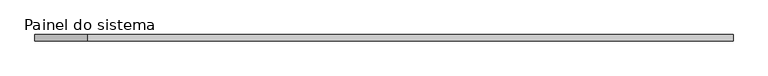
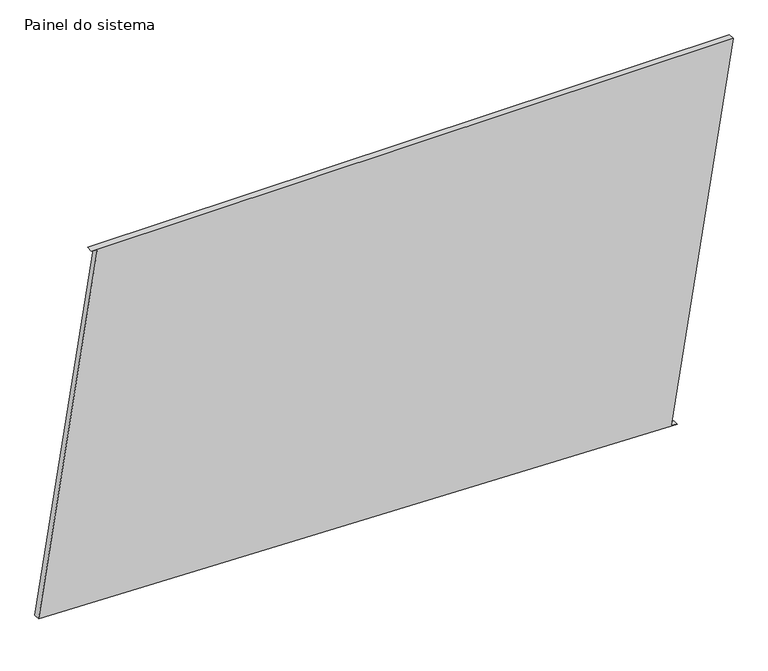
"""IFC4 building model written with IfcOpenShell, lengths in millimetres: plate geometry, Painel do sistema : Envidraçado."""

from ifc_helpers import new_model, si_unit, frame, origin, place, context, project, spatial, polyline, outline, extrude, source, transform, mapped, element, save


def painel_do_sistema_55de0004(model_context):
    return source(origin(), model_context, "Body", "SweptSolid", [
        extrude(outline(polyline([(0.0, 1172.2853497), (3.9380954, 1147.59747), (1560.8980645, 1395.9564583), (1560.8980645, -1183.881267), (1556.9599692, -1159.1933873), (72.6946874, -1395.9564583), (0.0, 1172.2853497)])), frame((0.0, 24.5, 0.0), z_axis=(0.0, 1.0, 0.0), x_axis=(0.0, 0.0, 1.0)), (0.0, 0.0, 1.0), 25.0),
    ])


if __name__ == "__main__":
    model = new_model("IFC4")
    model_context = context("Model", 3, world=origin())
    ifc_project = project(units=[si_unit("LENGTHUNIT", "METRE", prefix="MILLI")], contexts=[model_context])
    site = spatial("IfcSite", under=ifc_project)
    building = spatial("IfcBuilding", under=site)
    placement = place(None, origin())
    painel_do_sistema_shape = painel_do_sistema_55de0004(model_context)
    element("IfcPlate", 1, ObjectType="Painel do sistema : Envidraçado", at=placement, inside=building, context=model_context, shape_type="MappedRepresentation", body=[
        mapped(painel_do_sistema_shape, transform((0.0, 0.0, 0.0), x_axis=(1.0, 0.0, 0.0), y_axis=(0.0, 1.0, 0.0), z_axis=(0.0, 0.0, 1.0))),
    ])
    save(model, "model.ifc")

# Revit data of these elements
# Type "Painel do sistema : Envidraçado"
#   Construction Type Id = "GSP4R"
#   Analytic Construction = "Vidraça única Pilkington 1/8 pol"
#   Visual Light Transmittance = 0.9
#   Solar Heat Gain Coefficient = 0.86
#   Heat Transfer Coefficient (U) = 6.7069 W/(m²·K)
# Element 1 (IfcPlate, "Painel do sistema : Envidraçado")
#   Materials on its faces: "Vidro"
# Materials
#   "Vidro": class "Vidro", colour RGB 0 128 192, transparency 0.9, Description = "Vidro de sílica", Cost = 0
